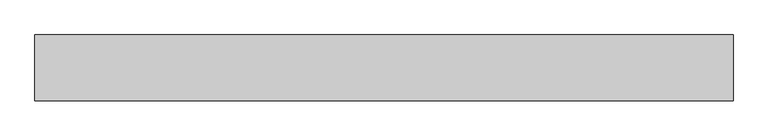
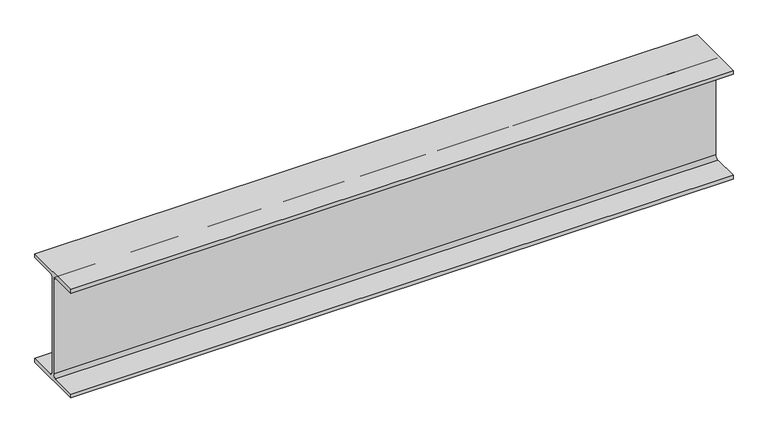
"""IFC4 building model written with IfcOpenShell, lengths in millimetres: beam geometry, Old_Steel Beam_H-KSD3502 : H_SB_ASB_H-482×300x11x15."""

from ifc_helpers import new_model, si_unit, point, frame, frame_2d, origin, place, context, project, spatial, polyline, circle_curve, trimmed, segment, composite_curve, outline, extrude, source, transform, mapped, element, save


def beam_6fec7774(model_context):
    return source(origin(), model_context, "Body", "SweptSolid", [
        extrude(outline(composite_curve([segment(polyline([(82.5, -141.5), (82.5, -151.7), (-82.5, -151.7), (-82.5, -141.5), (-11.9, -141.5)]), True, "CONTINUOUS"), segment(trimmed(circle_curve(frame_2d((-11.9, -132.6)), 8.9), [point((-11.9, -141.5))], [point((-3.0, -132.6))], True, "CARTESIAN"), True, "CONTINUOUS"), segment(polyline([(-3.0, -132.6), (-3.0, 132.6)]), True, "CONTINUOUS"), segment(trimmed(circle_curve(frame_2d((-11.9, 132.6)), 8.9), [point((-3.0, 132.6))], [point((-11.9, 141.5))], True, "CARTESIAN"), True, "CONTINUOUS"), segment(polyline([(-11.9, 141.5), (-82.5, 141.5), (-82.5, 151.7), (82.5, 151.7), (82.5, 141.5), (11.9, 141.5)]), True, "CONTINUOUS"), segment(trimmed(circle_curve(frame_2d((11.9, 132.6)), 8.9), [point((11.9, 141.5))], [point((3.0, 132.6))], True, "CARTESIAN"), True, "CONTINUOUS"), segment(polyline([(3.0, 132.6), (3.0, -132.6)]), True, "CONTINUOUS"), segment(trimmed(circle_curve(frame_2d((11.9, -132.6)), 8.9), [point((3.0, -132.6))], [point((11.9, -141.5))], True, "CARTESIAN"), True, "CONTINUOUS"), segment(polyline([(11.9, -141.5), (82.5, -141.5)]), True, "CONTINUOUS")], self_intersect=False)), frame((-870.3, 0.0, 0.0), z_axis=(1.0, 0.0, 0.0), x_axis=(0.0, 1.0, 0.0)), (0.0, 0.0, 1.0), 1753.3),
    ])


if __name__ == "__main__":
    model = new_model("IFC4")
    model_context = context("Model", 3, world=origin())
    ifc_project = project(units=[si_unit("LENGTHUNIT", "METRE", prefix="MILLI")], contexts=[model_context])
    site = spatial("IfcSite", under=ifc_project)
    building = spatial("IfcBuilding", under=site)
    placement = place(None, origin())
    beam_shape = beam_6fec7774(model_context)
    element("IfcBeam", 1, ObjectType="Old_Steel Beam_H-KSD3502 : H_SB_ASB_H-482×300x11x15", at=placement, inside=building, context=model_context, shape_type="MappedRepresentation", body=[
        mapped(beam_shape, transform((0.0, 0.0, 0.0), x_axis=(1.0, 0.0, 0.0), y_axis=(0.0, 1.0, 0.0), z_axis=(0.0, 0.0, 1.0))),
    ])
    save(model, "model.ifc")

# Revit data of these elements
# Type "Old_Steel Beam_H-KSD3502 : H_SB_ASB_H-482×300x11x15"
#   Width = 30.0 cm
#   Web Thickness = 1.1 cm
#   Web Fillet = 2.6 cm
#   Warping Constant = 3680250.0 cm⁶
#   Torsional Moment of Inertia = 88.2192 cm⁴
#   Torsional Modulus = 1.0 cm³
#   Section Area = 145.5 cm²
#   Plastic Modulus weak axis = 695.0 cm³
#   Plastic Modulus strong axis = 2790.0 cm³
#   Perimeter = 2.10 m²/m
#   Nominal Weight = 114.00 kgf/m
#   Moment of Inertia weak axis = 6760.00 cm⁴
#   Moment of Inertia strong axis = 60400.00 cm⁴
#   Height = 48.2 cm
#   Flange Thickness = 1.5 cm
#   Elastic Modulus weak axis = 451.0 cm³
#   Elastic Modulus strong axis = 2500.0 cm³
#   Centroid Vertical = 24.1 cm
#   Centroid Horizontal = 15.0 cm
#   Length [instance default] = 1.5240 m
#   Structural Material [instance default] = Steel, 45-345
#   Assembly Code = ""
# Element 1 (IfcBeam, "Old_Steel Beam_H-KSD3502 : H_SB_ASB_H-482×300x11x15")
#   Structural Material = none
# Materials
#   "Steel, 45-345": class "Metal", colour RGB 189 187 185, transparency 0, Description = "Steel 345 MPa", Cost = 0
